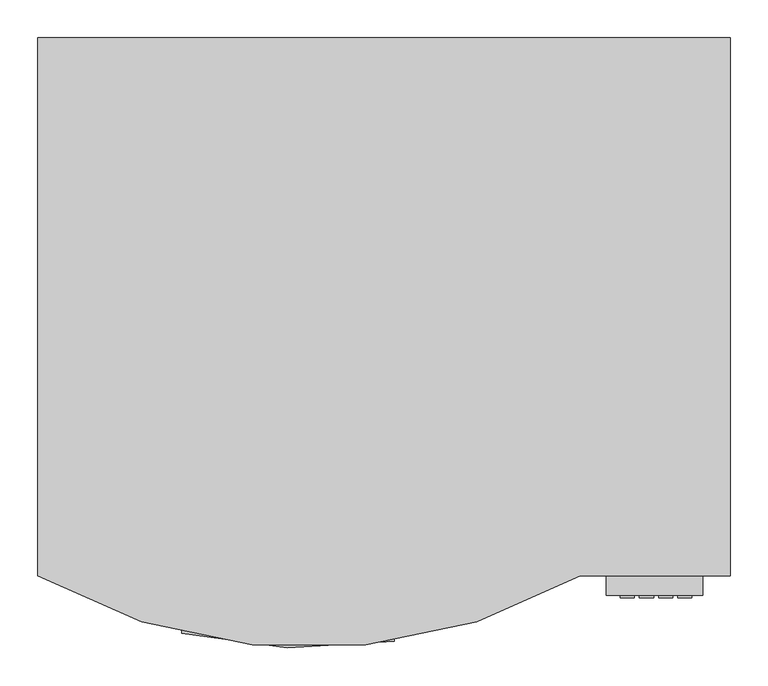
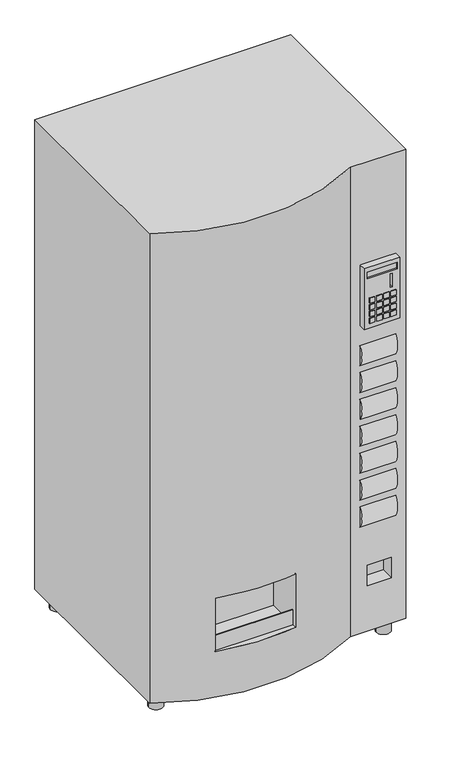
"""IFC4 building model written with IfcOpenShell, lengths in millimetres: proxy geometry, Getränkeautomat : Getränkeautomat."""

import ifcopenshell
import ifcopenshell.guid

model = None  # the IFC model being written
_history = None  # IfcOwnerHistory: only IFC2X3 demands one
_inside = {}  # id of a spatial element -> (the spatial element, [elements in it])
_under = {}  # id of a project, library or spatial element -> (it, [spatial elements below it])
_declared = {}  # id of a project -> (the project, [libraries it declares])
_typed = {}  # id of a type object -> (the type object, [elements of that type])
_made_of = {}  # id of a material, layer set ... -> (it, [elements and type objects made of it])


def new_model(schema):
    """Start an empty IFC model of exactly this schema.

    Asked for "IFC4X3", IfcOpenShell would pick the latest addendum, in which some entities
    have other attributes; the version numbers below select the first issue.
    IFC2X3 requires an IfcOwnerHistory on every rooted entity: one is made here for all.
    """
    global model, _history
    if schema == "IFC4X3":
        model = ifcopenshell.file(schema_version=(4, 3, 0, 0))
    else:
        model = ifcopenshell.file(schema=schema)
    _inside.clear()
    _under.clear()
    _declared.clear()
    _typed.clear()
    _made_of.clear()
    _history = None
    if model.schema == "IFC2X3":
        org = make("IfcOrganization", Name="unknown")
        user = make(
            "IfcPersonAndOrganization",
            ThePerson=make("IfcPerson", FamilyName="unknown"),
            TheOrganization=org,
        )
        app = make(
            "IfcApplication",
            ApplicationDeveloper=org,
            Version="unknown",
            ApplicationFullName="unknown",
            ApplicationIdentifier="unknown",
        )
        _history = make(
            "IfcOwnerHistory",
            OwningUser=user,
            OwningApplication=app,
            ChangeAction="ADDED",
            CreationDate=0,
        )
    return model


def make(cls, **values):
    """One entity of the class cls with the attributes given. An attribute that is None is left unset."""
    return model.create_entity(
        cls, **{name: value for name, value in values.items() if value is not None}
    )


def rooted(cls, **values):
    """An entity with a GlobalId (a new one), such as an element, a storey or a relation."""
    return make(cls, GlobalId=ifcopenshell.guid.new(), OwnerHistory=_history, **values)


def si_unit(unit_type, name, prefix=None):
    """IfcSIUnit, for example si_unit("LENGTHUNIT", "METRE", prefix="MILLI")."""
    return make("IfcSIUnit", UnitType=unit_type, Prefix=prefix, Name=name)


def assignment(units):
    """IfcUnitAssignment: the units of a project."""
    return None if units is None else make("IfcUnitAssignment", Units=units)


def point(xyz):
    """IfcCartesianPoint."""
    return None if xyz is None else make("IfcCartesianPoint", Coordinates=xyz)


def direction(xyz):
    """IfcDirection."""
    return None if xyz is None else make("IfcDirection", DirectionRatios=xyz)


def frame(location, z_axis=None, x_axis=None):
    """IfcAxis2Placement3D, a coordinate frame: its origin and axes. An axis left out is left unset."""
    return make(
        "IfcAxis2Placement3D",
        Location=point(location),
        Axis=direction(z_axis),
        RefDirection=direction(x_axis),
    )


def frame_2d(location, x_axis=None):
    """IfcAxis2Placement2D, a coordinate frame in the plane: its origin and x axis."""
    return make(
        "IfcAxis2Placement2D", Location=point(location), RefDirection=direction(x_axis)
    )


def origin():
    """The frame at (0, 0, 0) with its axes left unset."""
    return frame((0.0, 0.0, 0.0))


def origin_with_axes():
    """The frame at (0, 0, 0) with the z axis (0, 0, 1) and the x axis (1, 0, 0) written out."""
    return frame((0.0, 0.0, 0.0), z_axis=(0.0, 0.0, 1.0), x_axis=(1.0, 0.0, 0.0))


def place(relative_to, where):
    """IfcLocalPlacement: puts the frame where relative to a parent placement (None: the world)."""
    return make(
        "IfcLocalPlacement", PlacementRelTo=relative_to, RelativePlacement=where
    )


def context(
    kind, dimensions, precision=None, world=None, true_north=None, identifier=None
):
    """IfcGeometricRepresentationContext, for example the 3D "Model" context."""
    return make(
        "IfcGeometricRepresentationContext",
        ContextIdentifier=identifier,
        ContextType=kind,
        CoordinateSpaceDimension=dimensions,
        Precision=precision,
        WorldCoordinateSystem=world,
        TrueNorth=true_north,
    )


def project(units=None, contexts=None):
    """IfcProject with its units and contexts."""
    return rooted(
        "IfcProject",
        Name="project",
        RepresentationContexts=contexts,
        UnitsInContext=assignment(units),
    )


def spatial(cls, under=None, at=None, **own):
    """A site, building, storey or space (cls), placed at a placement, below another one or the project."""
    s = rooted(cls, ObjectPlacement=at, **own)
    if under is not None:
        _under.setdefault(under.id(), (under, []))[1].append(s)
    return s


def polyline(points):
    """IfcPolyline through the points."""
    return make("IfcPolyline", Points=[point(p) for p in points])


def circle_curve(where, radius):
    """IfcCircle in the frame where."""
    return make("IfcCircle", Position=where, Radius=radius)


def trimmed(basis, trim1, trim2, sense, master):
    """IfcTrimmedCurve: the piece of a basis curve between two trims."""
    return make(
        "IfcTrimmedCurve",
        BasisCurve=basis,
        Trim1=trim1,
        Trim2=trim2,
        SenseAgreement=sense,
        MasterRepresentation=master,
    )


def segment(curve, same_sense, transition):
    """IfcCompositeCurveSegment."""
    return make(
        "IfcCompositeCurveSegment",
        Transition=transition,
        SameSense=same_sense,
        ParentCurve=curve,
    )


def composite_curve(segments, self_intersect=None):
    """IfcCompositeCurve: segments joined end to end."""
    return make("IfcCompositeCurve", Segments=segments, SelfIntersect=self_intersect)


def outline(outer, holes=None, kind="AREA"):
    """IfcArbitraryClosedProfileDef: a profile drawn as a closed curve; with holes, ...WithVoids."""
    if holes is None:
        return make("IfcArbitraryClosedProfileDef", ProfileType=kind, OuterCurve=outer)
    return make(
        "IfcArbitraryProfileDefWithVoids",
        ProfileType=kind,
        OuterCurve=outer,
        InnerCurves=holes,
    )


def extrude(swept, where, along, depth):
    """IfcExtrudedAreaSolid: the profile swept, set in the frame where, extruded along a direction by depth."""
    return make(
        "IfcExtrudedAreaSolid",
        SweptArea=swept,
        Position=where,
        ExtrudedDirection=direction(along),
        Depth=depth,
    )


def faces_of(points, faces, orient=None, outer=None):
    """IfcFace entities. A face is a list of loops; a loop is a list of indices into points, from 0.

    orient and outer hold one flag for each loop. By default every Orientation is true, the
    first loop of a face is its IfcFaceOuterBound and the others are IfcFaceBound.
    """
    made = []
    for i, loops in enumerate(faces):
        bounds = []
        for j, loop in enumerate(loops):
            is_outer = j == 0 if outer is None else outer[i][j]
            bounds.append(
                make(
                    "IfcFaceOuterBound" if is_outer else "IfcFaceBound",
                    Bound=make("IfcPolyLoop", Polygon=[points[k] for k in loop]),
                    Orientation=True if orient is None else orient[i][j],
                )
            )
        made.append(make("IfcFace", Bounds=bounds))
    return made


def faceted_brep(points, faces, orient=None, outer=None, voids=None):
    """IfcFacetedBrep: a solid bounded by flat faces; with voids (closed shells), ...WithVoids."""
    shared = [point(p) for p in points]
    hull = make("IfcClosedShell", CfsFaces=faces_of(shared, faces, orient, outer))
    if voids is None:
        return make("IfcFacetedBrep", Outer=hull)
    return make(
        "IfcFacetedBrepWithVoids",
        Outer=hull,
        Voids=[
            make(cls, CfsFaces=faces_of(shared, fs, o, b)) for cls, fs, o, b in voids
        ],
    )


def shape(context_of_items, identifier, shape_type, items):
    """IfcShapeRepresentation: the items that make up one representation, for example the "Body"."""
    return make(
        "IfcShapeRepresentation",
        ContextOfItems=context_of_items,
        RepresentationIdentifier=identifier,
        RepresentationType=shape_type,
        Items=items,
    )


def source(mapping_origin, context_of_items, identifier, shape_type, items):
    """IfcRepresentationMap: a shape defined once, which mapped items show again and again."""
    return make(
        "IfcRepresentationMap",
        MappingOrigin=mapping_origin,
        MappedRepresentation=shape(context_of_items, identifier, shape_type, items),
    )


def transform(
    local_origin,
    x_axis=None,
    y_axis=None,
    z_axis=None,
    scale=None,
    scale2=None,
    scale3=None,
    uniform=True,
):
    """IfcCartesianTransformationOperator3D, or its non-uniform kind. x_axis, y_axis, z_axis: its Axis1, 2, 3."""
    if uniform:
        return make(
            "IfcCartesianTransformationOperator3D",
            Axis1=direction(x_axis),
            Axis2=direction(y_axis),
            LocalOrigin=point(local_origin),
            Scale=scale,
            Axis3=direction(z_axis),
        )
    return make(
        "IfcCartesianTransformationOperator3DnonUniform",
        Axis1=direction(x_axis),
        Axis2=direction(y_axis),
        LocalOrigin=point(local_origin),
        Scale=scale,
        Axis3=direction(z_axis),
        Scale2=scale2,
        Scale3=scale3,
    )


def mapped(mapping_source, mapping_target):
    """IfcMappedItem: shows the shape of a source again, moved by a transform."""
    return make(
        "IfcMappedItem", MappingSource=mapping_source, MappingTarget=mapping_target
    )


def made_of(thing, what):
    """Note that an element or type object is made of a material, layer set ...; save() writes the relation."""
    if what is not None:
        _made_of.setdefault(what.id(), (what, []))[1].append(thing)
    return thing


def element(
    cls,
    number,
    at=None,
    inside=None,
    cuts=None,
    type_object=None,
    material=None,
    context=None,
    identifier="Body",
    shape_type=None,
    held_by="IfcProductDefinitionShape",
    body=None,
    shapes=None,
    **own,
):
    """One element of the class cls, such as IfcWall. Its Tag is "e" and its number.

    at: its placement. inside: the storey or other place that contains it. cuts: it is an
    opening in that element (IfcRelVoidsElement). A single representation is given by context,
    identifier, shape_type and body (its items); several are given by shapes. held_by: the class
    of the entity that holds the representations. save() writes the other relations.
    """
    e = rooted(cls, Tag="e%d" % number, ObjectPlacement=at, **own)
    if body is not None:
        shapes = [shape(context, identifier, shape_type, body)]
    if shapes is not None:
        e.Representation = make(held_by, Representations=shapes)
    if inside is not None:
        _inside.setdefault(inside.id(), (inside, []))[1].append(e)
    if cuts is not None:
        rooted(
            "IfcRelVoidsElement", RelatingBuildingElement=cuts, RelatedOpeningElement=e
        )
    if type_object is not None:
        _typed.setdefault(type_object.id(), (type_object, []))[1].append(e)
    return made_of(e, material)


def aggregate(whole, parts):
    """IfcRelAggregates: a whole, such as a stair, and the parts it consists of."""
    return rooted("IfcRelAggregates", RelatingObject=whole, RelatedObjects=parts)


def save(model, path):
    """Write the relations noted so far, then the file.

    IfcRelAggregates (storeys below a building ...), IfcRelContainedInSpatialStructure (elements
    in a storey), IfcRelDefinesByType, IfcRelAssociatesMaterial and IfcRelDeclares: one each for
    every whole, place, type object, material and project.
    """
    for whole, parts in _under.values():
        aggregate(whole, parts)
    for where, things in _inside.values():
        rooted(
            "IfcRelContainedInSpatialStructure",
            RelatedElements=things,
            RelatingStructure=where,
        )
    for kind, things in _typed.values():
        rooted("IfcRelDefinesByType", RelatedObjects=things, RelatingType=kind)
    for what, things in _made_of.values():
        rooted("IfcRelAssociatesMaterial", RelatedObjects=things, RelatingMaterial=what)
    for by, libraries in _declared.values():
        rooted("IfcRelDeclares", RelatingContext=by, RelatedDefinitions=libraries)
    model.write(path)


def plane_surface(at):
    """IfcPlane: the flat surface through the origin of the frame at, square to its z axis."""
    return make("IfcPlane", Position=at)


def cylinder_surface(at, radius):
    """IfcCylindricalSurface: all points at the distance radius from the z axis of the frame at."""
    return make("IfcCylindricalSurface", Position=at, Radius=radius)


def advanced_brep(points, edges, surfaces, faces):
    """IfcAdvancedBrep: a solid bounded by faces that lie on surfaces and meet in shared edges.

    An edge is (start, end): straight between two places in points (the first is 0);
    or (start, end, curve); or (start, end, curve, False) where it runs against its curve.
    A face is (place in surfaces, loops), or (place, loops, False) where it looks against
    its surface's normal. A loop lists edges by number (the first is 1), with a minus sign
    where the edge is run from its end to its start. The first loop is the outer one.
    """
    corners = [point(p) for p in points]
    vertices = [make("IfcVertexPoint", VertexGeometry=c) for c in corners]
    made = []
    for start, end, *more in edges:
        made.append(
            make(
                "IfcEdgeCurve",
                EdgeStart=vertices[start],
                EdgeEnd=vertices[end],
                EdgeGeometry=more[0] if more else make("IfcPolyline", Points=[corners[start], corners[end]]),
                SameSense=more[1] if len(more) > 1 else True,
            )
        )
    hull = []
    for where, loops, *sense in faces:
        bounds = []
        for j, loop in enumerate(loops):
            ring = [make("IfcOrientedEdge", EdgeElement=made[abs(k) - 1], Orientation=k > 0) for k in loop]
            bounds.append(
                make(
                    "IfcFaceOuterBound" if j == 0 else "IfcFaceBound",
                    Bound=make("IfcEdgeLoop", EdgeList=ring),
                    Orientation=True,
                )
            )
        hull.append(make("IfcAdvancedFace", Bounds=bounds, FaceSurface=surfaces[where], SameSense=sense[0] if sense else True))
    return make("IfcAdvancedBrep", Outer=make("IfcClosedShell", CfsFaces=hull))


def specialty_equipment_d6c7ff97(model_context):
    return source(origin(), model_context, "Body", "SolidModel", [
        extrude(outline(composite_curve([segment(trimmed(circle_curve(frame_2d((-216.0902216, 1105.4279487)), 67.5221597), [point((-271.8363609, 1067.3279487))], [point((-271.8363609, 1143.5279487))], False, "CARTESIAN"), True, "CONTINUOUS"), segment(polyline([(-271.8363609, 1143.5279487), (-271.8363609, 1067.3279487)]), True, "CONTINUOUS")], self_intersect=False)), frame((275.3159229, 0.0, 0.0), z_axis=(1.0, 0.0, 0.0), x_axis=(0.0, 1.0, 0.0)), (0.0, 0.0, 1.0), 127.0948963),
        extrude(outline(composite_curve([segment(trimmed(circle_curve(frame_2d((-216.0902216, 1003.8279487)), 67.5221597), [point((-271.8363609, 965.7279487))], [point((-271.8363609, 1041.9279487))], False, "CARTESIAN"), True, "CONTINUOUS"), segment(polyline([(-271.8363609, 1041.9279487), (-271.8363609, 965.7279487)]), True, "CONTINUOUS")], self_intersect=False)), frame((275.3159229, 0.0, 0.0), z_axis=(1.0, 0.0, 0.0), x_axis=(0.0, 1.0, 0.0)), (0.0, 0.0, 1.0), 127.0948963),
        extrude(outline(composite_curve([segment(trimmed(circle_curve(frame_2d((-216.0902216, 902.2279487)), 67.5221597), [point((-271.8363609, 864.1279487))], [point((-271.8363609, 940.3279487))], False, "CARTESIAN"), True, "CONTINUOUS"), segment(polyline([(-271.8363609, 940.3279487), (-271.8363609, 864.1279487)]), True, "CONTINUOUS")], self_intersect=False)), frame((275.3159229, 0.0, 0.0), z_axis=(1.0, 0.0, 0.0), x_axis=(0.0, 1.0, 0.0)), (0.0, 0.0, 1.0), 127.0948963),
        extrude(outline(composite_curve([segment(trimmed(circle_curve(frame_2d((-216.0902216, 800.6279487)), 67.5221597), [point((-271.8363609, 762.5279487))], [point((-271.8363609, 838.7279487))], False, "CARTESIAN"), True, "CONTINUOUS"), segment(polyline([(-271.8363609, 838.7279487), (-271.8363609, 762.5279487)]), True, "CONTINUOUS")], self_intersect=False)), frame((275.3159229, 0.0, 0.0), z_axis=(1.0, 0.0, 0.0), x_axis=(0.0, 1.0, 0.0)), (0.0, 0.0, 1.0), 127.0948963),
        extrude(outline(composite_curve([segment(trimmed(circle_curve(frame_2d((-216.0902216, 699.0279487)), 67.5221597), [point((-271.8363609, 660.9279487))], [point((-271.8363609, 737.1279487))], False, "CARTESIAN"), True, "CONTINUOUS"), segment(polyline([(-271.8363609, 737.1279487), (-271.8363609, 660.9279487)]), True, "CONTINUOUS")], self_intersect=False)), frame((275.3159229, 0.0, 0.0), z_axis=(1.0, 0.0, 0.0), x_axis=(0.0, 1.0, 0.0)), (0.0, 0.0, 1.0), 127.0948963),
        extrude(outline(composite_curve([segment(trimmed(circle_curve(frame_2d((-216.0902216, 597.4279487)), 67.5221597), [point((-271.8363609, 559.3279487))], [point((-271.8363609, 635.5279487))], False, "CARTESIAN"), True, "CONTINUOUS"), segment(polyline([(-271.8363609, 635.5279487), (-271.8363609, 559.3279487)]), True, "CONTINUOUS")], self_intersect=False)), frame((275.3159229, 0.0, 0.0), z_axis=(1.0, 0.0, 0.0), x_axis=(0.0, 1.0, 0.0)), (0.0, 0.0, 1.0), 127.0948963),
        extrude(outline(composite_curve([segment(trimmed(circle_curve(frame_2d((-216.0902216, 495.8279487)), 67.5221597), [point((-271.8363609, 457.7279487))], [point((-271.8363609, 533.9279487))], False, "CARTESIAN"), True, "CONTINUOUS"), segment(polyline([(-271.8363609, 533.9279487), (-271.8363609, 457.7279487)]), True, "CONTINUOUS")], self_intersect=False)), frame((275.3159229, 0.0, 0.0), z_axis=(1.0, 0.0, 0.0), x_axis=(0.0, 1.0, 0.0)), (0.0, 0.0, 1.0), 127.0948963),
        faceted_brep([(402.3159229, -297.2363609, 1448.3279487), (275.3159229, -297.2363609, 1448.3279487), (275.3159229, -297.2363609, 1219.7279487), (402.3159229, -297.2363609, 1219.7279487), (286.3445758, -297.2363609, 1432.5207795), (394.2945758, -297.2363609, 1432.5207795), (394.2945758, -297.2363609, 1407.1207795), (286.3445758, -297.2363609, 1407.1207795), (369.009172, -297.2363609, 1397.7730022), (375.359172, -297.2363609, 1397.7730022), (375.359172, -297.2363609, 1346.9730022), (369.009172, -297.2363609, 1346.9730022), (402.3159229, -271.8363609, 1448.3279487), (402.3159229, -271.8363609, 1219.7279487), (275.3159229, -271.8363609, 1219.7279487), (275.3159229, -271.8363609, 1448.3279487), (394.2945758, -290.8863609, 1432.5207795), (286.3445758, -290.8863609, 1432.5207795), (286.3445758, -290.8863609, 1407.1207795), (394.2945758, -290.8863609, 1407.1207795), (375.359172, -275.0113609, 1397.7730022), (369.009172, -275.0113609, 1397.7730022), (369.009172, -275.0113609, 1346.9730022), (375.359172, -275.0113609, 1346.9730022)], [[[0, 1, 2, 3], [4, 5, 6, 7], [8, 9, 10, 11]], [[12, 13, 14, 15]], [[1, 0, 12, 15]], [[2, 1, 15, 14]], [[3, 2, 14, 13]], [[0, 3, 13, 12]], [[16, 17, 18, 19]], [[17, 16, 5, 4]], [[18, 17, 4, 7]], [[19, 18, 7, 6]], [[16, 19, 6, 5]], [[20, 21, 22, 23]], [[21, 20, 9, 8]], [[22, 21, 8, 11]], [[23, 22, 11, 10]], [[20, 23, 10, 9]]]),
        extrude(outline(polyline([(-4.9505365, -342.4801109), (-285.8560243, -342.4801109), (-285.8560243, -339.3678837), (-4.9505365, -339.3678837), (-4.9505365, -342.4801109)])), frame((0.0, 0.0, 227.0552601), z_axis=(0.0, 0.0, 1.0), x_axis=(1.0, 0.0, 0.0)), (0.0, 0.0, 1.0), 59.7862005),
        extrude(outline(composite_curve([segment(trimmed(circle_curve(frame_2d((-424.8751183, 388.5636391)), 25.4), [point((-450.2751183, 388.5636391))], [point((-399.4751183, 388.5636391))], False, "CARTESIAN"), True, "CONTINUOUS"), segment(trimmed(circle_curve(frame_2d((-424.8751183, 388.5636391)), 25.4), [point((-399.4751183, 388.5636391))], [point((-450.2751183, 388.5636391))], False, "CARTESIAN"), True, "CONTINUOUS")], self_intersect=False)), origin_with_axes(), (0.0, 0.0, 1.0), 55.5625),
        extrude(outline(composite_curve([segment(trimmed(circle_curve(frame_2d((387.9248817, 388.5636391)), 25.4), [point((362.5248817, 388.5636391))], [point((413.3248817, 388.5636391))], False, "CARTESIAN"), True, "CONTINUOUS"), segment(trimmed(circle_curve(frame_2d((387.9248817, 388.5636391)), 25.4), [point((413.3248817, 388.5636391))], [point((362.5248817, 388.5636391))], False, "CARTESIAN"), True, "CONTINUOUS")], self_intersect=False)), origin_with_axes(), (0.0, 0.0, 1.0), 55.5625),
        extrude(outline(composite_curve([segment(trimmed(circle_curve(frame_2d((387.9248817, -221.0363609)), 25.4), [point((362.5248817, -221.0363609))], [point((413.3248817, -221.0363609))], False, "CARTESIAN"), True, "CONTINUOUS"), segment(trimmed(circle_curve(frame_2d((387.9248817, -221.0363609)), 25.4), [point((413.3248817, -221.0363609))], [point((362.5248817, -221.0363609))], False, "CARTESIAN"), True, "CONTINUOUS")], self_intersect=False)), origin_with_axes(), (0.0, 0.0, 1.0), 55.5625),
        extrude(outline(composite_curve([segment(trimmed(circle_curve(frame_2d((-424.8751183, -221.0363609)), 25.4), [point((-450.2751183, -221.0363609))], [point((-399.4751183, -221.0363609))], False, "CARTESIAN"), True, "CONTINUOUS"), segment(trimmed(circle_curve(frame_2d((-424.8751183, -221.0363609)), 25.4), [point((-399.4751183, -221.0363609))], [point((-450.2751183, -221.0363609))], False, "CARTESIAN"), True, "CONTINUOUS")], self_intersect=False)), origin_with_axes(), (0.0, 0.0, 1.0), 55.5625),
        advanced_brep(
        [(438.7248817, 439.3636391, 1828.8), (-475.6751183, 439.3636391, 1828.8), (-475.6751183, -271.8363609, 1828.8), (240.962407, -271.8363609, 1828.8), (438.7248817, -271.8363609, 1828.8), (438.7248817, 439.3636391, 55.4895962), (438.7248817, -271.8363609, 55.4895962), (240.962407, -271.8363609, 55.4895962), (-475.6751183, -271.8363609, 55.4895962), (-475.6751183, 439.3636391, 55.4895962), (-285.8560243, -347.1225541, 431.8), (-4.9505365, -358.2607189, 431.8), (-4.9505365, -358.2607189, 229.9895559), (-285.8560243, -347.1225541, 229.9895559), (387.9248817, -271.8363609, 304.8), (387.9248817, -271.8363609, 227.0552601), (301.300731, -271.8363609, 227.0552601), (301.300731, -271.8363609, 304.8), (-4.9505365, -221.0363609, 431.8), (-285.8560243, -221.0363609, 431.8), (-285.8560243, -221.0363609, 229.9895559), (-4.9505365, -221.0363609, 229.9895559), (387.9248817, -221.0363609, 304.8), (301.300731, -221.0363609, 304.8), (301.300731, -221.0363609, 227.0552601), (387.9248817, -221.0363609, 227.0552601)],
        [
            (0, 1),
            (1, 2),
            (2, 3, circle_curve(frame((-117.3563557, 354.6542517, 1828.8), z_axis=(0.0, 0.0, 1.0), x_axis=(1.0, 0.0, 0.0)), 721.7221234)),
            (3, 4),
            (4, 0),
            (5, 6),
            (6, 7),
            (7, 8, circle_curve(frame((-117.3563557, 354.6542517, 55.4895962), z_axis=(0.0, 0.0, -1.0), x_axis=(1.0, 0.0, 0.0)), 721.7221234)),
            (8, 9),
            (9, 5),
            (0, 5),
            (9, 1),
            (8, 2),
            (7, 3),
            (10, 11, circle_curve(frame((-117.3563557, 354.6542517, 431.8), z_axis=(0.0, 0.0, 1.0), x_axis=(1.0, 0.0, 0.0)), 721.7221234)),
            (11, 12),
            (12, 13, circle_curve(frame((-117.3563557, 354.6542517, 229.9895559), z_axis=(0.0, 0.0, -1.0), x_axis=(1.0, 0.0, 0.0)), 721.7221234)),
            (13, 10),
            (6, 4),
            (14, 15),
            (15, 16),
            (16, 17),
            (17, 14),
            (18, 19),
            (19, 20),
            (20, 21),
            (21, 18),
            (18, 11),
            (10, 19),
            (13, 20),
            (12, 21),
            (22, 23),
            (23, 24),
            (24, 25),
            (25, 22),
            (25, 15),
            (14, 22),
            (24, 16),
            (23, 17),
        ],
        [
            plane_surface(frame((-475.6751183, 439.3636391, 1828.8), z_axis=(0.0, 0.0, 1.0), x_axis=(-1.0, 0.0, 0.0))),
            plane_surface(frame((-475.6751183, 439.3636391, 55.4895962), z_axis=(0.0, 0.0, -1.0), x_axis=(1.0, 0.0, 0.0))),
            plane_surface(frame((438.7248817, 439.3636391, 1828.8), z_axis=(0.0, 1.0, 0.0), x_axis=(0.0, 0.0, -1.0))),
            plane_surface(frame((-475.6751183, 439.3636391, 1828.8), z_axis=(-1.0, 0.0, 0.0), x_axis=(0.0, 0.0, -1.0))),
            cylinder_surface(frame((-117.3563557, 354.6542517, 55.4895962), z_axis=(0.0, 0.0, 1.0), x_axis=(1.0, 0.0, 0.0)), 721.7221234),
            plane_surface(frame((240.962407, -271.8363609, 1828.8), z_axis=(0.0, -1.0, 0.0), x_axis=(0.0, 0.0, -1.0))),
            plane_surface(frame((438.7248817, -271.8363609, 1828.8), z_axis=(1.0, 0.0, 0.0), x_axis=(0.0, 0.0, -1.0))),
            plane_surface(frame((-285.8560243, -221.0363609, 431.8), z_axis=(0.0, -1.0, 0.0), x_axis=(1.0, 0.0, 0.0))),
            plane_surface(frame((-4.9505365, -383.6604873, 431.8), z_axis=(0.0, 0.0, -1.0), x_axis=(0.0, 1.0, 0.0))),
            plane_surface(frame((-285.8560243, -383.6604873, 431.8), z_axis=(1.0, 0.0, 0.0), x_axis=(0.0, 1.0, 0.0))),
            plane_surface(frame((-285.8560243, -383.6604873, 229.9895559), z_axis=(0.0, 0.0, 1.0), x_axis=(0.0, 1.0, 0.0))),
            plane_surface(frame((-4.9505365, -383.6604873, 229.9895559), z_axis=(-1.0, 0.0, 0.0), x_axis=(0.0, 1.0, 0.0))),
            plane_surface(frame((387.9248817, -221.0363609, 304.8), z_axis=(0.0, -1.0, 0.0), x_axis=(0.0, 0.0, -1.0))),
            plane_surface(frame((387.9248817, -221.0363609, 304.8), z_axis=(-1.0, 0.0, 0.0), x_axis=(0.0, -1.0, 0.0))),
            plane_surface(frame((387.9248817, -221.0363609, 227.0552601), z_axis=(0.0, 0.0, 1.0), x_axis=(0.0, -1.0, 0.0))),
            plane_surface(frame((301.300731, -221.0363609, 227.0552601), z_axis=(1.0, 0.0, 0.0), x_axis=(0.0, -1.0, 0.0))),
            plane_surface(frame((301.300731, -221.0363609, 304.8), z_axis=(0.0, 0.0, -1.0), x_axis=(0.0, -1.0, 0.0))),
        ],
        [
            (0, [[1, 2, 3, 4, 5]]),
            (1, [[6, 7, 8, 9, 10]]),
            (2, [[-1, 11, -10, 12]]),
            (3, [[-2, -12, -9, 13]]),
            (4, [[-3, -13, -8, 14], [15, 16, 17, 18]]),
            (5, [[-4, -14, -7, 19], [20, 21, 22, 23]]),
            (6, [[-5, -19, -6, -11]]),
            (7, [[24, 25, 26, 27]]),
            (8, [[-24, 28, -15, 29]]),
            (9, [[-25, -29, -18, 30]]),
            (10, [[-26, -30, -17, 31]]),
            (11, [[-27, -31, -16, -28]]),
            (12, [[32, 33, 34, 35]]),
            (13, [[-35, 36, -20, 37]]),
            (14, [[-34, 38, -21, -36]]),
            (15, [[-33, 39, -22, -38]]),
            (16, [[-32, -37, -23, -39]]),
        ],
    ),
        extrude(outline(polyline([(312.3802372, -300.4113609), (293.3302372, -300.4113609), (293.3302372, -297.2363609), (312.3802372, -297.2363609), (312.3802372, -300.4113609)])), frame((0.0, 0.0, 1313.6452473), z_axis=(0.0, 0.0, 1.0), x_axis=(1.0, 0.0, 0.0)), (0.0, 0.0, 1.0), 19.05),
        extrude(outline(polyline([(312.3802372, -300.4113609), (293.3302372, -300.4113609), (293.3302372, -297.2363609), (312.3802372, -297.2363609), (312.3802372, -300.4113609)])), frame((0.0, 0.0, 1237.4452473), z_axis=(0.0, 0.0, 1.0), x_axis=(1.0, 0.0, 0.0)), (0.0, 0.0, 1.0), 19.05),
        extrude(outline(polyline([(387.9248817, -300.4113609), (369.5302372, -300.4113609), (369.5302372, -297.2363609), (387.9248817, -297.2363609), (387.9248817, -300.4113609)])), frame((0.0, 0.0, 1237.4452473), z_axis=(0.0, 0.0, 1.0), x_axis=(1.0, 0.0, 0.0)), (0.0, 0.0, 1.0), 19.05),
        extrude(outline(polyline([(387.9248817, -300.4113609), (369.5302372, -300.4113609), (369.5302372, -297.2363609), (387.9248817, -297.2363609), (387.9248817, -300.4113609)])), frame((0.0, 0.0, 1313.6452473), z_axis=(0.0, 0.0, 1.0), x_axis=(1.0, 0.0, 0.0)), (0.0, 0.0, 1.0), 19.05),
        extrude(outline(polyline([(312.3802372, -300.4113609), (293.3302372, -300.4113609), (293.3302372, -297.2363609), (312.3802372, -297.2363609), (312.3802372, -300.4113609)])), frame((0.0, 0.0, 1288.2452473), z_axis=(0.0, 0.0, 1.0), x_axis=(1.0, 0.0, 0.0)), (0.0, 0.0, 1.0), 19.05),
        extrude(outline(polyline([(312.3802372, -300.4113609), (293.3302372, -300.4113609), (293.3302372, -297.2363609), (312.3802372, -297.2363609), (312.3802372, -300.4113609)])), frame((0.0, 0.0, 1262.8452473), z_axis=(0.0, 0.0, 1.0), x_axis=(1.0, 0.0, 0.0)), (0.0, 0.0, 1.0), 19.05),
        extrude(outline(polyline([(337.7802372, -300.4113609), (318.7302372, -300.4113609), (318.7302372, -297.2363609), (337.7802372, -297.2363609), (337.7802372, -300.4113609)])), frame((0.0, 0.0, 1313.6452473), z_axis=(0.0, 0.0, 1.0), x_axis=(1.0, 0.0, 0.0)), (0.0, 0.0, 1.0), 19.05),
        extrude(outline(polyline([(363.1802372, -300.4113609), (344.1302372, -300.4113609), (344.1302372, -297.2363609), (363.1802372, -297.2363609), (363.1802372, -300.4113609)])), frame((0.0, 0.0, 1313.6452473), z_axis=(0.0, 0.0, 1.0), x_axis=(1.0, 0.0, 0.0)), (0.0, 0.0, 1.0), 19.05),
        extrude(outline(polyline([(337.7802372, -300.4113609), (318.7302372, -300.4113609), (318.7302372, -297.2363609), (337.7802372, -297.2363609), (337.7802372, -300.4113609)])), frame((0.0, 0.0, 1237.4452473), z_axis=(0.0, 0.0, 1.0), x_axis=(1.0, 0.0, 0.0)), (0.0, 0.0, 1.0), 19.05),
        extrude(outline(polyline([(363.1802372, -300.4113609), (344.1302372, -300.4113609), (344.1302372, -297.2363609), (363.1802372, -297.2363609), (363.1802372, -300.4113609)])), frame((0.0, 0.0, 1237.4452473), z_axis=(0.0, 0.0, 1.0), x_axis=(1.0, 0.0, 0.0)), (0.0, 0.0, 1.0), 19.05),
        extrude(outline(polyline([(387.9248817, -300.4113609), (369.5302372, -300.4113609), (369.5302372, -297.2363609), (387.9248817, -297.2363609), (387.9248817, -300.4113609)])), frame((0.0, 0.0, 1262.8452473), z_axis=(0.0, 0.0, 1.0), x_axis=(1.0, 0.0, 0.0)), (0.0, 0.0, 1.0), 19.05),
        extrude(outline(polyline([(387.9248817, -300.4113609), (369.5302372, -300.4113609), (369.5302372, -297.2363609), (387.9248817, -297.2363609), (387.9248817, -300.4113609)])), frame((0.0, 0.0, 1288.2452473), z_axis=(0.0, 0.0, 1.0), x_axis=(1.0, 0.0, 0.0)), (0.0, 0.0, 1.0), 19.05),
        extrude(outline(polyline([(337.7802372, -300.4113609), (318.7302372, -300.4113609), (318.7302372, -297.2363609), (337.7802372, -297.2363609), (337.7802372, -300.4113609)])), frame((0.0, 0.0, 1262.8452473), z_axis=(0.0, 0.0, 1.0), x_axis=(1.0, 0.0, 0.0)), (0.0, 0.0, 1.0), 19.05),
        extrude(outline(polyline([(363.1802372, -300.4113609), (344.1302372, -300.4113609), (344.1302372, -297.2363609), (363.1802372, -297.2363609), (363.1802372, -300.4113609)])), frame((0.0, 0.0, 1262.8452473), z_axis=(0.0, 0.0, 1.0), x_axis=(1.0, 0.0, 0.0)), (0.0, 0.0, 1.0), 19.05),
        extrude(outline(polyline([(363.1802372, -300.4113609), (344.1302372, -300.4113609), (344.1302372, -297.2363609), (363.1802372, -297.2363609), (363.1802372, -300.4113609)])), frame((0.0, 0.0, 1288.2452473), z_axis=(0.0, 0.0, 1.0), x_axis=(1.0, 0.0, 0.0)), (0.0, 0.0, 1.0), 19.05),
        extrude(outline(polyline([(337.7802372, -300.4113609), (318.7302372, -300.4113609), (318.7302372, -297.2363609), (337.7802372, -297.2363609), (337.7802372, -300.4113609)])), frame((0.0, 0.0, 1288.2452473), z_axis=(0.0, 0.0, 1.0), x_axis=(1.0, 0.0, 0.0)), (0.0, 0.0, 1.0), 19.05),
    ])


if __name__ == "__main__":
    model = new_model("IFC4")
    model_context = context("Model", 3, world=origin())
    ifc_project = project(units=[si_unit("LENGTHUNIT", "METRE", prefix="MILLI")], contexts=[model_context])
    site = spatial("IfcSite", under=ifc_project)
    building = spatial("IfcBuilding", under=site)
    placement = place(None, origin())
    specialty_equipment_shape = specialty_equipment_d6c7ff97(model_context)
    element("IfcBuildingElementProxy", 1, Name="Getränkeautomat : Getränkeautomat", ObjectType="Getränkeautomat : Getränkeautomat", at=placement, inside=building, context=model_context, shape_type="MappedRepresentation", body=[
        mapped(specialty_equipment_shape, transform((0.0, 0.0, 0.0), x_axis=(1.0, 0.0, 0.0), y_axis=(0.0, 1.0, 0.0), z_axis=(0.0, 0.0, 1.0))),
    ])
    save(model, "model.ifc")

# Revit data of these elements
# Type "Getränkeautomat : Getränkeautomat"
#   Assembly Code = ""
# Element 1 (IfcBuildingElementProxy, "Getränkeautomat : Getränkeautomat")
#   Materials on its faces: "Metall - Edelstahl", "Kunststoff - Braun", "Metall - Stahl"
# Materials
#   "Metall - Edelstahl": class "Metall", colour RGB 176 176 176, transparency 0
#   "Kunststoff - Braun": class "Kunststoff", colour RGB 176 109 71, transparency 0
#   "Metall - Stahl": class "Metall", colour RGB 247 247 247, transparency 0, Cost = 0
